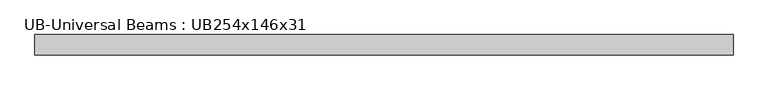
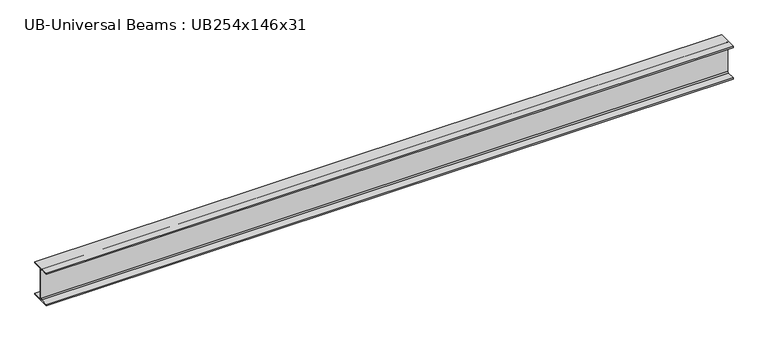
"""IFC4 building model written with IfcOpenShell, lengths in millimetres: beam geometry, UB-Universal Beams : UB254x146x31."""

from ifc_helpers import new_model, si_unit, point, frame, frame_2d, origin, place, context, project, spatial, polyline, circle_curve, trimmed, segment, composite_curve, outline, extrude, source, transform, mapped, element, save


def ub_universal_beams_ub254x146x31_ce116be2(model_context):
    return source(origin(), model_context, "Body", "SweptSolid", [
        extrude(outline(composite_curve([segment(polyline([(73.05, -117.1), (73.05, -125.7), (-73.05, -125.7), (-73.05, -117.1), (-10.6, -117.1)]), True, "CONTINUOUS"), segment(trimmed(circle_curve(frame_2d((-10.6, -109.5)), 7.6), [point((-10.6, -117.1))], [point((-3.0, -109.5))], True, "CARTESIAN"), True, "CONTINUOUS"), segment(polyline([(-3.0, -109.5), (-3.0, 109.5)]), True, "CONTINUOUS"), segment(trimmed(circle_curve(frame_2d((-10.6, 109.5)), 7.6), [point((-3.0, 109.5))], [point((-10.6, 117.1))], True, "CARTESIAN"), True, "CONTINUOUS"), segment(polyline([(-10.6, 117.1), (-73.05, 117.1), (-73.05, 125.7), (73.05, 125.7), (73.05, 117.1), (10.6, 117.1)]), True, "CONTINUOUS"), segment(trimmed(circle_curve(frame_2d((10.6, 109.5)), 7.6), [point((10.6, 117.1))], [point((3.0, 109.5))], True, "CARTESIAN"), True, "CONTINUOUS"), segment(polyline([(3.0, 109.5), (3.0, -109.5)]), True, "CONTINUOUS"), segment(trimmed(circle_curve(frame_2d((10.6, -109.5)), 7.6), [point((3.0, -109.5))], [point((10.6, -117.1))], True, "CARTESIAN"), True, "CONTINUOUS"), segment(polyline([(10.6, -117.1), (73.05, -117.1)]), True, "CONTINUOUS")], self_intersect=False)), frame((-2500.0, 0.0, 0.0), z_axis=(1.0, 0.0, 0.0), x_axis=(0.0, 1.0, 0.0)), (0.0, 0.0, 1.0), 5000.0),
    ])


if __name__ == "__main__":
    model = new_model("IFC4")
    model_context = context("Model", 3, world=origin())
    ifc_project = project(units=[si_unit("LENGTHUNIT", "METRE", prefix="MILLI")], contexts=[model_context])
    site = spatial("IfcSite", under=ifc_project)
    building = spatial("IfcBuilding", under=site)
    placement = place(None, origin())
    ub_universal_beams_ub254x146x31_shape = ub_universal_beams_ub254x146x31_ce116be2(model_context)
    element("IfcBeam", 1, ObjectType="UB-Universal Beams : UB254x146x31", at=placement, inside=building, context=model_context, shape_type="MappedRepresentation", body=[
        mapped(ub_universal_beams_ub254x146x31_shape, transform((0.0, 0.0, 0.0), x_axis=(1.0, 0.0, 0.0), y_axis=(0.0, 1.0, 0.0), z_axis=(0.0, 0.0, 1.0))),
    ])
    save(model, "model.ifc")

# Revit data of these elements
# Type "UB-Universal Beams : UB254x146x31"
#   Section Name Key = "UB254X146X31"
#   Width = 14.61 cm
#   Web Thickness = 0.6 cm
#   Web Fillet = 0.76 cm
#   Warping Constant = 66000.0 cm⁶
#   Torsional Moment of Inertia = 8.55 cm⁴
#   Section Area = 39.7 cm²
#   Plastic Modulus weak axis = 94.1 cm³
#   Plastic Modulus strong axis = 393.0 cm³
#   Nominal Weight = 31.10 kgf/m
#   Moment of Inertia weak axis = 448.00 cm⁴
#   Moment of Inertia strong axis = 4413.00 cm⁴
#   Height = 25.14 cm
#   Flange Thickness = 0.86 cm
#   Elastic Modulus weak axis = 61.3 cm³
#   Elastic Modulus strong axis = 351.0 cm³
#   Centroid Vertical = 12.57 cm
#   Centroid Horizontal = 7.305 cm
#   Bolt Spacing = 7.0 cm
#   Length [instance default] = 1500 mm
#   Structural Material [instance default] = Metal - Steel 43-275
#   Type Comments = ""
#   Assembly Code = ""
# Element 1 (IfcBeam, "UB-Universal Beams : UB254x146x31")
#   Materials on its faces: "Metal - Steel 43-275"
# Materials
#   "Metal - Steel 43-275": class "Metal", colour RGB 247 247 247, transparency 0, Cost = 0
